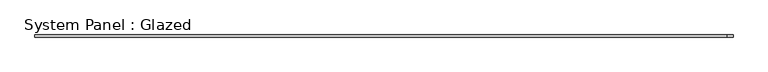
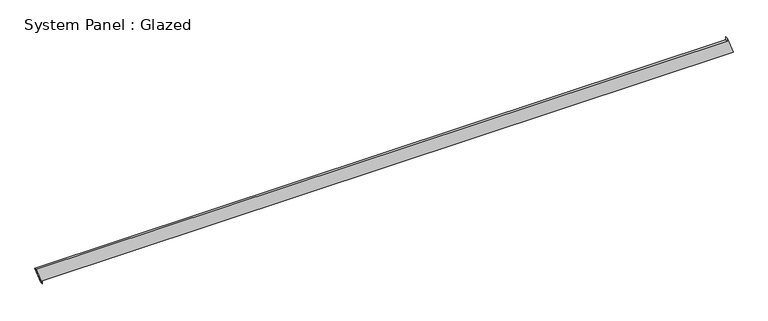
"""IFC4 building model written with IfcOpenShell, lengths in millimetres: plate geometry, System Panel : Glazed."""

from ifc_helpers import new_model, si_unit, frame, origin, place, context, project, spatial, polyline, outline, extrude, source, transform, mapped, element, save


def system_panel_glazed_db2940a7(model_context):
    return source(origin(), model_context, "Body", "SweptSolid", [
        extrude(outline(polyline([(0.0, -3958.4484867), (35.3553391, -3958.4484867), (35.3553391, 4028.4582851), (235.1502568, 3958.3300218), (199.7949178, 3958.329801), (199.8448074, -4028.4582851), (0.0, -3958.4484867)])), frame((0.0, -49.5, 0.0), z_axis=(0.0, 1.0, 0.0), x_axis=(0.0, 0.0, 1.0)), (0.0, 0.0, 1.0), 25.0),
    ])


if __name__ == "__main__":
    model = new_model("IFC4")
    model_context = context("Model", 3, world=origin())
    ifc_project = project(units=[si_unit("LENGTHUNIT", "METRE", prefix="MILLI")], contexts=[model_context])
    site = spatial("IfcSite", under=ifc_project)
    building = spatial("IfcBuilding", under=site)
    placement = place(None, origin())
    system_panel_glazed_shape = system_panel_glazed_db2940a7(model_context)
    element("IfcPlate", 1, ObjectType="System Panel : Glazed", at=placement, inside=building, context=model_context, shape_type="MappedRepresentation", body=[
        mapped(system_panel_glazed_shape, transform((0.0, 0.0, 0.0), x_axis=(1.0, 0.0, 0.0), y_axis=(0.0, 1.0, 0.0), z_axis=(0.0, 0.0, 1.0))),
    ])
    save(model, "model.ifc")

# Revit data of these elements
# Element 1 (IfcPlate, "System Panel : Glazed")
#   Materials on its faces: "Glass"
# Materials
#   "Glass": class "Glass", colour RGB 218 227 224, transparency 0.85, Description = "Soda Lime Glass", Cost = 0
